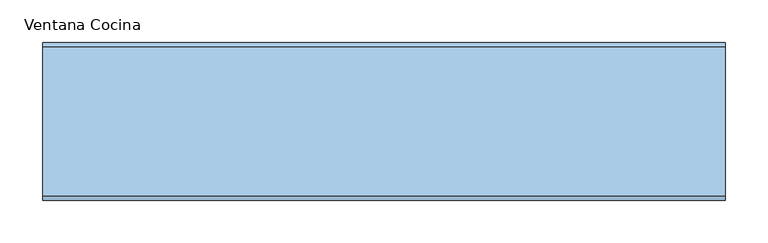
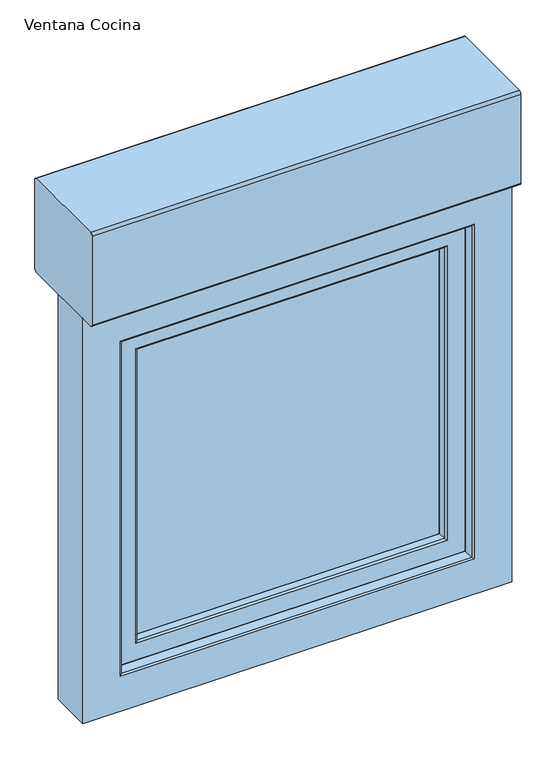
"""IFC4 building model written with IfcOpenShell, lengths in millimetres: window geometry, 2019_ES_Ventana_Replus_re80pvc301_10100_box_1-Hoja_con-Compacto : Ventana Cocina."""

from ifc_helpers import new_model, si_unit, point, frame, frame_2d, origin, place, context, project, spatial, polyline, circle_curve, ellipse_curve, trimmed, segment, composite_curve, outline, extrude, source, transform, mapped, element, save
from ifc_brep_helpers import plane_surface, cylinder_surface, advanced_brep


def ventana_cocina_83fcc546(model_context):
    return source(origin(), model_context, "Body", "SolidModel", [
        extrude(outline(composite_curve([segment(trimmed(circle_curve(frame_2d((-55.0, 1615.0)), 5.0), [point((-55.0, 1610.0))], [point((-60.0, 1615.0))], False, "CARTESIAN"), True, "CONTINUOUS"), segment(polyline([(-60.0, 1615.0), (-60.0, 1790.0)]), True, "CONTINUOUS"), segment(trimmed(circle_curve(frame_2d((-55.0, 1790.0)), 5.0), [point((-60.0, 1790.0))], [point((-55.0, 1795.0))], False, "CARTESIAN"), True, "CONTINUOUS"), segment(polyline([(-55.0, 1795.0), (120.0, 1795.0)]), True, "CONTINUOUS"), segment(trimmed(circle_curve(frame_2d((120.0, 1790.0)), 5.0), [point((120.0, 1795.0))], [point((125.0, 1790.0))], False, "CARTESIAN"), True, "CONTINUOUS"), segment(polyline([(125.0, 1790.0), (125.0, 1615.0)]), True, "CONTINUOUS"), segment(trimmed(circle_curve(frame_2d((120.0, 1615.0)), 5.0), [point((125.0, 1615.0))], [point((120.0, 1610.0))], False, "CARTESIAN"), True, "CONTINUOUS"), segment(polyline([(120.0, 1610.0), (-55.0, 1610.0)]), True, "CONTINUOUS")], self_intersect=False)), frame((-400.0, 0.0, 0.0), z_axis=(1.0, 0.0, 0.0), x_axis=(0.0, 1.0, 0.0)), (0.0, 0.0, 1.0), 800.0),
        extrude(outline(polyline([(78.4999991, 1420.0), (118.4999991, 1420.0), (118.4999991, 1310.0), (98.4999991, 1310.0), (98.4999991, 1400.0), (78.4999991, 1400.0), (78.4999991, 1420.0)])), frame((-334.1999993, 0.0, 0.0), z_axis=(1.0, 0.0, 0.0), x_axis=(0.0, 1.0, 0.0)), (0.0, 0.0, 1.0), 12.0),
        extrude(outline(polyline([(-313.9687607, 78.4999991), (-313.9687607, 68.4999991), (-342.4312378, 68.4999991), (-342.4312378, 78.4999991), (-313.9687607, 78.4999991)])), frame((0.0, 0.0, 1385.217127), z_axis=(0.0, 0.0, 1.0), x_axis=(1.0, 0.0, 0.0)), (0.0, 0.0, 1.0), 49.565746),
        extrude(outline(polyline([(909.8, 297.1999993), (1507.2, 297.1999993), (1507.2, -297.1999993), (909.8, -297.1999993), (909.8, 297.1999993)]), holes=[polyline([(1499.2, 289.1999993), (917.8, 289.1999993), (917.8, -289.1999993), (1499.2, -289.1999993), (1499.2, 289.1999993)])]), frame((0.0, 10.9999999, 0.0), z_axis=(0.0, 1.0, 0.0), x_axis=(0.0, 0.0, 1.0)), (0.0, 0.0, 1.0), 16.0),
        extrude(outline(polyline([(909.8131934, 297.1868058), (1507.1868066, 297.1868058), (1507.1868066, -297.1868058), (909.8131934, -297.1868058), (909.8131934, 297.1868058)]), holes=[polyline([(1499.2, 289.1999993), (917.8, 289.1999993), (917.8, -289.1999993), (1499.2, -289.1999993), (1499.2, 289.1999993)])]), frame((0.0, 31.0000001, 0.0), z_axis=(0.0, 1.0, 0.0), x_axis=(0.0, 0.0, 1.0)), (0.0, 0.0, 1.0), 16.0),
        extrude(outline(polyline([(297.1999993, 6.9999997), (-297.1999993, 6.9999997), (-297.1999993, 10.9999999), (297.1999993, 10.9999999), (297.1999993, 6.9999997)])), frame((0.0, 0.0, 903.7946451), z_axis=(0.0, 0.0, 1.0), x_axis=(1.0, 0.0, 0.0)), (0.0, 0.0, 1.0), 609.4053549),
        extrude(outline(polyline([(297.1999993, 26.9999999), (-297.1999993, 26.9999999), (-297.1999993, 31.0000001), (297.1999993, 31.0000001), (297.1999993, 26.9999999)])), frame((0.0, 0.0, 903.7946451), z_axis=(0.0, 0.0, 1.0), x_axis=(1.0, 0.0, 0.0)), (0.0, 0.0, 1.0), 609.4053549),
        extrude(outline(polyline([(297.1999993, 47.0000001), (-297.1999993, 47.0000001), (-297.1999993, 51.0000003), (297.1999993, 51.0000003), (297.1999993, 47.0000001)])), frame((0.0, 0.0, 903.7946451), z_axis=(0.0, 0.0, 1.0), x_axis=(1.0, 0.0, 0.0)), (0.0, 0.0, 1.0), 609.4053549),
        advanced_brep(
        [(287.2913171, -9.2764571, 1497.2913178), (287.2913171, -9.2764571, 922.7086822), (290.1890946, -11.5, 919.8109047), (290.1890946, -11.5, 1500.1890953), (330.1999993, -11.5, 879.8), (330.1999993, -11.5, 1540.2), (-330.1999993, -11.5, 1540.2), (-330.1999993, -11.5, 879.8), (-290.1890946, -11.5, 919.8109047), (-290.1890946, -11.5, 1500.1890953), (-287.2913171, -9.2764571, 922.7086822), (284.1757968, 2.3508228, 1494.1757976), (284.1757968, 2.3508228, 925.8242024), (-284.1757968, 2.3508228, 925.8242024), (284.6739305, 3.0000033, 1494.6739313), (284.6739305, 3.0000033, 925.3260687), (-284.6739305, 3.0000033, 925.3260687), (291.1999993, 3.0000033, 1501.2), (291.1999993, 3.0000033, 918.8), (-291.1999993, 3.0000033, 918.8), (-291.1999993, 3.0000033, 1501.2), (-284.6739305, 3.0000033, 1494.6739313), (291.1999993, 6.9999997, 1501.2), (291.1999993, 6.9999997, 918.8), (-291.1999993, 6.9999997, 918.8), (311.8162192, 6.9999997, 1521.8162199), (311.8162192, 6.9999997, 898.1837801), (-311.8162192, 6.9999997, 898.1837801), (-311.8162192, 6.9999997, 1521.8162199), (-291.1999993, 6.9999997, 1501.2), (309.1999993, 25.6153717, 1519.2), (309.1999993, 25.6153717, 900.8), (-309.1999993, 25.6153717, 900.8), (309.1999993, 56.4999995, 1519.2), (309.1999993, 56.4999995, 900.8), (-309.1999993, 56.4999995, 900.8), (-309.1999993, 56.4999995, 1519.2), (297.1999993, 56.4999995, 1507.2), (297.1999993, 56.4999995, 912.8), (-297.1999993, 56.4999995, 912.8), (-297.1999993, 56.4999995, 1507.2), (297.1999993, 51.0000003, 1507.2), (297.1999993, 51.0000003, 912.8), (-297.1999993, 51.0000003, 912.8), (-297.1999993, 51.0000003, 1507.2), (286.007687, 51.0000003, 1496.0076877), (286.007687, 51.0000003, 923.9923123), (-286.007687, 51.0000003, 923.9923123), (-286.007687, 51.0000003, 1496.0076877), (285.4940999, 51.6693201, 1495.4941006), (285.4940999, 51.6693201, 924.5058994), (-285.4940999, 51.6693201, 924.5058994), (288.8993918, 64.3780426, 1498.8993925), (288.8993918, 64.3780426, 921.1006075), (-288.8993918, 64.3780426, 921.1006075), (292.6234971, 67.3403297, 1502.6234978), (292.6234971, 67.3403297, 917.3765022), (-292.6234971, 67.3403297, 917.3765022), (305.6488427, 67.7951848, 1515.6488434), (305.6488427, 67.7951848, 904.3511566), (-305.6488427, 67.7951848, 904.3511566), (306.1999993, 67.2629391, 1516.2), (306.1999993, 67.2629391, 903.8), (-306.1999993, 67.2629391, 903.8), (307.4370593, 68.4999991, 1517.43706), (307.4370593, 68.4999991, 902.56294), (-307.4370593, 68.4999991, 902.56294), (360.1999993, 68.4999991, 1570.2), (360.1999993, 68.4999991, 849.8), (-360.1999993, 68.4999991, 849.8), (-360.1999993, 68.4999991, 1570.2), (-307.4370593, 68.4999991, 1517.43706), (363.1999993, 65.4999991, 1573.2), (363.1999993, 65.4999991, 846.8), (-363.1999993, 65.4999991, 846.8), (363.1999993, 50.0, 1573.2), (363.1999993, 50.0, 846.8), (-363.1999993, 50.0, 846.8), (-363.1999993, 50.0, 1573.2), (343.1999993, 50.0, 1553.2), (343.1999993, 50.0, 866.8), (-343.1999993, 50.0, 866.8), (-343.1999993, 50.0, 1553.2), (343.1999993, 11.9999991, 1553.2), (343.1999993, 11.9999991, 866.8), (-343.1999993, 11.9999991, 866.8), (-343.1999993, 11.9999991, 1553.2), (330.1999993, 11.9999991, 1540.2), (330.1999993, 11.9999991, 879.8), (-330.1999993, 11.9999991, 879.8), (-330.1999993, 11.9999991, 1540.2), (-287.2913171, -9.2764571, 1497.2913178), (-284.1757968, 2.3508228, 1494.1757976), (-309.1999993, 25.6153717, 1519.2), (-285.4940999, 51.6693201, 1495.4941006), (-288.8993918, 64.3780426, 1498.8993925), (-292.6234971, 67.3403297, 1502.6234978), (-305.6488427, 67.7951848, 1515.6488434), (-306.1999993, 67.2629391, 1516.2), (-363.1999993, 65.4999991, 1573.2)],
        [
            (0, 1),
            (1, 2, ellipse_curve(frame((290.1890946, -8.5, 919.8109047), z_axis=(0.7071067811865475, 0.0, 0.7071067811865475), x_axis=(-0.7071067811865474, 0.0, 0.7071067811865476)), 4.2426407, 3.0)),
            (2, 3),
            (3, 0, ellipse_curve(frame((290.1890946, -8.5, 1500.1890953), z_axis=(0.7071067811865475, 0.0, -0.7071067811865475), x_axis=(0.7071067811865474, 0.0, 0.7071067811865476)), 4.2426407, 3.0)),
            (4, 5),
            (5, 6),
            (6, 7),
            (7, 4),
            (2, 8),
            (8, 9),
            (9, 3),
            (1, 10),
            (10, 8, ellipse_curve(frame((-290.1890946, -8.5, 919.8109047), z_axis=(0.7071067811865475, 0.0, -0.7071067811865475), x_axis=(0.7071067811865476, 0.0, 0.7071067811865474)), 4.2426407, 3.0)),
            (11, 12),
            (12, 1),
            (0, 11),
            (12, 13),
            (13, 10),
            (14, 15),
            (15, 12, ellipse_curve(frame((284.6739305, 2.4842973, 925.3260687), z_axis=(0.7071067811865475, 0.0, 0.7071067811865475), x_axis=(-0.7071067811865474, 0.0, 0.7071067811865476)), 0.7293184, 0.515706)),
            (11, 14, ellipse_curve(frame((284.6739305, 2.4842973, 1494.6739313), z_axis=(0.7071067811865475, 0.0, -0.7071067811865475), x_axis=(0.7071067811865474, 0.0, 0.7071067811865476)), 0.7293184, 0.515706)),
            (15, 16),
            (16, 13, ellipse_curve(frame((-284.6739305, 2.4842973, 925.3260687), z_axis=(0.7071067811865475, 0.0, -0.7071067811865475), x_axis=(0.7071067811865476, 0.0, 0.7071067811865474)), 0.7293184, 0.515706)),
            (17, 18),
            (18, 19),
            (19, 20),
            (20, 17),
            (14, 21),
            (21, 16),
            (22, 23),
            (23, 18),
            (17, 22),
            (23, 24),
            (24, 19),
            (25, 26),
            (26, 27),
            (27, 28),
            (28, 25),
            (22, 29),
            (29, 24),
            (30, 31),
            (31, 26),
            (25, 30),
            (31, 32),
            (32, 27),
            (33, 34),
            (34, 31),
            (30, 33),
            (34, 35),
            (35, 32),
            (33, 36),
            (36, 35),
            (37, 38),
            (38, 39),
            (39, 40),
            (40, 37),
            (41, 42),
            (42, 38),
            (37, 41),
            (42, 43),
            (43, 39),
            (41, 44),
            (44, 43),
            (45, 46),
            (46, 47),
            (47, 48),
            (48, 45),
            (49, 50),
            (50, 46, ellipse_curve(frame((286.007687, 51.5317048, 923.9923123), z_axis=(0.7071067811865475, 0.0, 0.7071067811865475), x_axis=(-0.7071067811865474, 0.0, 0.7071067811865476)), 0.7519437, 0.5317045)),
            (45, 49, ellipse_curve(frame((286.007687, 51.5317048, 1496.0076877), z_axis=(0.7071067811865475, 0.0, -0.7071067811865475), x_axis=(0.7071067811865474, 0.0, 0.7071067811865476)), 0.7519437, 0.5317045)),
            (50, 51),
            (51, 47, ellipse_curve(frame((-286.007687, 51.5317048, 923.9923123), z_axis=(0.7071067811865475, 0.0, -0.7071067811865475), x_axis=(0.7071067811865476, 0.0, 0.7071067811865474)), 0.7519437, 0.5317045)),
            (52, 53),
            (53, 50),
            (49, 52),
            (53, 54),
            (54, 51),
            (55, 56),
            (56, 53, ellipse_curve(frame((292.7630951, 63.3427664, 917.2369042), z_axis=(0.7071067811865475, 0.0, 0.7071067811865475), x_axis=(-0.7071067811865474, 0.0, 0.7071067811865476)), 5.6568542, 4.0)),
            (52, 55, ellipse_curve(frame((292.7630951, 63.3427664, 1502.7630958), z_axis=(0.7071067811865475, 0.0, -0.7071067811865475), x_axis=(0.7071067811865474, 0.0, 0.7071067811865476)), 5.6568542, 4.0)),
            (56, 57),
            (57, 54, ellipse_curve(frame((-292.7630951, 63.3427664, 917.2369042), z_axis=(0.7071067811865475, 0.0, -0.7071067811865475), x_axis=(0.7071067811865476, 0.0, 0.7071067811865474)), 5.6568542, 4.0)),
            (58, 59),
            (59, 56),
            (55, 58),
            (59, 60),
            (60, 57),
            (61, 62),
            (62, 59, ellipse_curve(frame((305.6674291, 67.2629391, 904.3325701), z_axis=(0.7071067811865475, 0.0, 0.7071067811865475), x_axis=(-0.7071067811865474, 0.0, 0.7071067811865476)), 0.7531679, 0.5325701)),
            (58, 61, ellipse_curve(frame((305.6674291, 67.2629391, 1515.6674299), z_axis=(0.7071067811865475, 0.0, -0.7071067811865475), x_axis=(0.7071067811865474, 0.0, 0.7071067811865476)), 0.7531679, 0.5325701)),
            (62, 63),
            (63, 60, ellipse_curve(frame((-305.6674291, 67.2629391, 904.3325701), z_axis=(0.7071067811865475, 0.0, -0.7071067811865475), x_axis=(0.7071067811865476, 0.0, 0.7071067811865474)), 0.7531679, 0.5325701)),
            (64, 65),
            (65, 62, ellipse_curve(frame((307.4370593, 67.2629391, 902.56294), z_axis=(0.7071067811865475, 0.0, 0.7071067811865475), x_axis=(-0.7071067811865474, 0.0, 0.7071067811865476)), 1.7494671, 1.23706)),
            (61, 64, ellipse_curve(frame((307.4370593, 67.2629391, 1517.43706), z_axis=(0.7071067811865475, 0.0, -0.7071067811865475), x_axis=(0.7071067811865474, 0.0, 0.7071067811865476)), 1.7494671, 1.23706)),
            (65, 66),
            (66, 63, ellipse_curve(frame((-307.4370593, 67.2629391, 902.56294), z_axis=(0.7071067811865475, 0.0, -0.7071067811865475), x_axis=(0.7071067811865476, 0.0, 0.7071067811865474)), 1.7494671, 1.23706)),
            (67, 68),
            (68, 69),
            (69, 70),
            (70, 67),
            (64, 71),
            (71, 66),
            (72, 73),
            (73, 68, ellipse_curve(frame((360.1999993, 65.4999991, 849.8), z_axis=(0.7071067811865475, 0.0, 0.7071067811865475), x_axis=(-0.7071067811865474, 0.0, 0.7071067811865476)), 4.2426407, 3.0)),
            (67, 72, ellipse_curve(frame((360.1999993, 65.4999991, 1570.2), z_axis=(0.7071067811865475, 0.0, -0.7071067811865475), x_axis=(0.7071067811865474, 0.0, 0.7071067811865476)), 4.2426407, 3.0)),
            (73, 74),
            (74, 69, ellipse_curve(frame((-360.1999993, 65.4999991, 849.8), z_axis=(0.7071067811865475, 0.0, -0.7071067811865475), x_axis=(0.7071067811865476, 0.0, 0.7071067811865474)), 4.2426407, 3.0)),
            (75, 76),
            (76, 73),
            (72, 75),
            (76, 77),
            (77, 74),
            (75, 78),
            (78, 77),
            (79, 80),
            (80, 81),
            (81, 82),
            (82, 79),
            (79, 83),
            (83, 84),
            (84, 80),
            (84, 85),
            (85, 81),
            (83, 86),
            (86, 85),
            (87, 88),
            (88, 89),
            (89, 90),
            (90, 87),
            (87, 5),
            (4, 88),
            (7, 89),
            (10, 91),
            (91, 9, ellipse_curve(frame((-290.1890946, -8.5, 1500.1890953), z_axis=(-0.7071067811865475, 0.0, -0.7071067811865475), x_axis=(0.7071067811865474, 0.0, -0.7071067811865476)), 4.2426407, 3.0)),
            (13, 92),
            (92, 91),
            (21, 92, ellipse_curve(frame((-284.6739305, 2.4842973, 1494.6739313), z_axis=(-0.7071067811865475, 0.0, -0.7071067811865475), x_axis=(0.7071067811865474, 0.0, -0.7071067811865476)), 0.7293184, 0.515706)),
            (29, 20),
            (32, 93),
            (93, 28),
            (36, 93),
            (44, 40),
            (51, 94),
            (94, 48, ellipse_curve(frame((-286.007687, 51.5317048, 1496.0076877), z_axis=(-0.7071067811865475, 0.0, -0.7071067811865475), x_axis=(0.7071067811865474, 0.0, -0.7071067811865476)), 0.7519437, 0.5317045)),
            (54, 95),
            (95, 94),
            (57, 96),
            (96, 95, ellipse_curve(frame((-292.7630951, 63.3427664, 1502.7630958), z_axis=(-0.7071067811865475, 0.0, -0.7071067811865475), x_axis=(0.7071067811865474, 0.0, -0.7071067811865476)), 5.6568542, 4.0)),
            (60, 97),
            (97, 96),
            (63, 98),
            (98, 97, ellipse_curve(frame((-305.6674291, 67.2629391, 1515.6674299), z_axis=(-0.7071067811865475, 0.0, -0.7071067811865475), x_axis=(0.7071067811865474, 0.0, -0.7071067811865476)), 0.7531679, 0.5325701)),
            (71, 98, ellipse_curve(frame((-307.4370593, 67.2629391, 1517.43706), z_axis=(-0.7071067811865475, 0.0, -0.7071067811865475), x_axis=(0.7071067811865474, 0.0, -0.7071067811865476)), 1.7494671, 1.23706)),
            (74, 99),
            (99, 70, ellipse_curve(frame((-360.1999993, 65.4999991, 1570.2), z_axis=(-0.7071067811865475, 0.0, -0.7071067811865475), x_axis=(0.7071067811865474, 0.0, -0.7071067811865476)), 4.2426407, 3.0)),
            (78, 99),
            (86, 82),
            (6, 90),
            (91, 0),
            (92, 11),
            (93, 30),
            (94, 49),
            (95, 52),
            (96, 55),
            (97, 58),
            (98, 61),
            (99, 72),
        ],
        [
            cylinder_surface(frame((290.1890946, -8.5, 1573.2), z_axis=(0.0, 0.0, 1.0), x_axis=(-1.0, 0.0, 0.0)), 3.0),
            plane_surface(frame((-330.1999993, -11.5, 1540.2), z_axis=(0.0, -1.0, 0.0), x_axis=(1.0, 0.0, 0.0))),
            cylinder_surface(frame((363.1999993, -8.5, 919.8109047), z_axis=(1.0, 0.0, 0.0), x_axis=(0.0, 0.0, 1.0)), 3.0),
            plane_surface(frame((287.2913171, -9.2764571, 1497.2913178), z_axis=(-0.9659258263570556, -0.258819044848789, 0.0), x_axis=(0.0, 0.0, -1.0))),
            plane_surface(frame((287.2913171, -9.2764571, 922.7086822), z_axis=(0.0, -0.2588190448487859, 0.9659258263570565), x_axis=(-1.0, 0.0, 0.0))),
            cylinder_surface(frame((284.6739305, 2.4842973, 1573.2), z_axis=(0.0, 0.0, 1.0), x_axis=(-1.0, 0.0, 0.0)), 0.515706),
            cylinder_surface(frame((363.1999993, 2.4842973, 925.3260687), z_axis=(1.0, 0.0, 0.0), x_axis=(0.0, 0.0, 1.0)), 0.515706),
            plane_surface(frame((-284.6739305, 3.0000033, 1494.6739313), z_axis=(0.0, 1.0, 0.0), x_axis=(1.0, 0.0, 0.0))),
            plane_surface(frame((291.1999993, 3.0000033, 1501.2), z_axis=(-1.0, 0.0, 0.0), x_axis=(0.0, 0.0, -1.0))),
            plane_surface(frame((291.1999993, 3.0000033, 918.8), z_axis=(0.0, 0.0, 1.0), x_axis=(-1.0, 0.0, 0.0))),
            plane_surface(frame((-291.1999993, 6.9999997, 1501.2), z_axis=(0.0, 1.0, 0.0), x_axis=(1.0, 0.0, 0.0))),
            plane_surface(frame((311.8162192, 6.9999997, 1521.8162199), z_axis=(-0.9902680687415736, -0.13917310096004265, 0.0), x_axis=(0.0, 0.0, -1.0))),
            plane_surface(frame((311.8162192, 6.9999997, 898.1837801), z_axis=(0.0, -0.13917310096003943, 0.990268068741574), x_axis=(-1.0, 0.0, 0.0))),
            plane_surface(frame((309.1999993, 25.6153717, 1519.2), z_axis=(-1.0, 0.0, 0.0), x_axis=(0.0, 0.0, -1.0))),
            plane_surface(frame((309.1999993, 25.6153717, 900.8), z_axis=(0.0, 0.0, 1.0), x_axis=(-1.0, 0.0, 0.0))),
            plane_surface(frame((-309.1999993, 56.4999995, 1519.2), z_axis=(0.0, -1.0, 0.0), x_axis=(1.0, 0.0, 0.0))),
            plane_surface(frame((297.1999993, 56.4999995, 1507.2), z_axis=(1.0, 0.0, 0.0), x_axis=(0.0, 0.0, -1.0))),
            plane_surface(frame((297.1999993, 56.4999995, 912.8), z_axis=(0.0, 0.0, -1.0), x_axis=(-1.0, 0.0, 0.0))),
            plane_surface(frame((-297.1999993, 51.0000003, 1507.2), z_axis=(0.0, -1.0, 0.0), x_axis=(1.0, 0.0, 0.0))),
            cylinder_surface(frame((286.007687, 51.5317048, 1573.2), z_axis=(0.0, 0.0, 1.0), x_axis=(-1.0, 0.0, 0.0)), 0.5317045),
            cylinder_surface(frame((363.1999993, 51.5317048, 923.9923123), z_axis=(1.0, 0.0, 0.0), x_axis=(0.0, 0.0, 1.0)), 0.5317045),
            plane_surface(frame((285.4940999, 51.6693201, 1495.4941006), z_axis=(-0.9659258262890666, 0.2588190451025272, 0.0), x_axis=(0.0, 0.0, -1.0))),
            plane_surface(frame((285.4940999, 51.6693201, 924.5058994), z_axis=(0.0, 0.2588190451025303, 0.9659258262890658), x_axis=(-1.0, 0.0, 0.0))),
            cylinder_surface(frame((292.7630951, 63.3427664, 1573.2), z_axis=(0.0, 0.0, 1.0), x_axis=(-1.0, 0.0, 0.0)), 4.0),
            cylinder_surface(frame((363.1999993, 63.3427664, 917.2369042), z_axis=(1.0, 0.0, 0.0), x_axis=(0.0, 0.0, 1.0)), 4.0),
            plane_surface(frame((292.6234971, 67.3403297, 1502.6234978), z_axis=(-0.03489949670250791, 0.9993908270190955, 0.0), x_axis=(0.0, 0.0, -1.0))),
            plane_surface(frame((292.6234971, 67.3403297, 917.3765022), z_axis=(0.0, 0.9993908270190957, 0.034899496702504675), x_axis=(-1.0, 0.0, 0.0))),
            cylinder_surface(frame((305.6674291, 67.2629391, 1573.2), z_axis=(0.0, 0.0, 1.0), x_axis=(-1.0, 0.0, 0.0)), 0.5325701),
            cylinder_surface(frame((363.1999993, 67.2629391, 904.3325701), z_axis=(1.0, 0.0, 0.0), x_axis=(0.0, 0.0, 1.0)), 0.5325701),
            cylinder_surface(frame((307.4370593, 67.2629391, 1573.2), z_axis=(0.0, 0.0, 1.0), x_axis=(-1.0, 0.0, 0.0)), 1.23706),
            cylinder_surface(frame((363.1999993, 67.2629391, 902.56294), z_axis=(1.0, 0.0, 0.0), x_axis=(0.0, 0.0, 1.0)), 1.23706),
            plane_surface(frame((-307.4370593, 68.4999991, 1517.43706), z_axis=(0.0, 1.0, 0.0), x_axis=(1.0, 0.0, 0.0))),
            cylinder_surface(frame((360.1999993, 65.4999991, 1573.2), z_axis=(0.0, 0.0, 1.0), x_axis=(-1.0, 0.0, 0.0)), 3.0),
            cylinder_surface(frame((363.1999993, 65.4999991, 849.8), z_axis=(1.0, 0.0, 0.0), x_axis=(0.0, 0.0, 1.0)), 3.0),
            plane_surface(frame((363.1999993, 65.4999991, 1573.2), z_axis=(1.0, 0.0, 0.0), x_axis=(0.0, 0.0, -1.0))),
            plane_surface(frame((363.1999993, 65.4999991, 846.8), z_axis=(0.0, 0.0, -1.0), x_axis=(-1.0, 0.0, 0.0))),
            plane_surface(frame((-359.2000019, 50.0, 1569.2000027), z_axis=(0.0, -1.0, 0.0), x_axis=(1.0, 0.0, 0.0))),
            plane_surface(frame((343.1999993, 45.0999991, 1553.2), z_axis=(1.0, 0.0, 0.0), x_axis=(0.0, 0.0, -1.0))),
            plane_surface(frame((343.1999993, 45.0999991, 866.8), z_axis=(0.0, 0.0, -1.0), x_axis=(-1.0, 0.0, 0.0))),
            plane_surface(frame((-335.7000002, 11.9999991, 1545.7000009), z_axis=(0.0, -1.0, 0.0), x_axis=(1.0, 0.0, 0.0))),
            plane_surface(frame((330.1999993, 1.4999991, 1540.2), z_axis=(1.0, 0.0, 0.0), x_axis=(0.0, 0.0, -1.0))),
            plane_surface(frame((330.1999993, 1.4999991, 879.8), z_axis=(0.0, 0.0, -1.0), x_axis=(-1.0, 0.0, 0.0))),
            cylinder_surface(frame((-290.1890946, -8.5, 846.8), z_axis=(0.0, 0.0, -1.0), x_axis=(1.0, 0.0, 0.0)), 3.0),
            plane_surface(frame((-287.2913171, -9.2764571, 922.7086822), z_axis=(0.9659258263570573, -0.25881904484878276, 0.0), x_axis=(0.0, 0.0, 1.0))),
            cylinder_surface(frame((-284.6739305, 2.4842973, 846.8), z_axis=(0.0, 0.0, -1.0), x_axis=(1.0, 0.0, 0.0)), 0.515706),
            plane_surface(frame((-291.1999993, 3.0000033, 918.8), z_axis=(1.0, 0.0, 0.0), x_axis=(0.0, 0.0, 1.0))),
            plane_surface(frame((-311.8162192, 6.9999997, 898.1837801), z_axis=(0.9902680687415745, -0.1391731009600362, 0.0), x_axis=(0.0, 0.0, 1.0))),
            plane_surface(frame((-309.1999993, 25.6153717, 900.8), z_axis=(1.0, 0.0, 0.0), x_axis=(0.0, 0.0, 1.0))),
            plane_surface(frame((-297.1999993, 56.4999995, 912.8), z_axis=(-1.0, 0.0, 0.0), x_axis=(0.0, 0.0, 1.0))),
            cylinder_surface(frame((-286.007687, 51.5317048, 846.8), z_axis=(0.0, 0.0, -1.0), x_axis=(1.0, 0.0, 0.0)), 0.5317045),
            plane_surface(frame((-285.4940999, 51.6693201, 924.5058994), z_axis=(0.9659258262890649, 0.2588190451025334, 0.0), x_axis=(0.0, 0.0, 1.0))),
            cylinder_surface(frame((-292.7630951, 63.3427664, 846.8), z_axis=(0.0, 0.0, -1.0), x_axis=(1.0, 0.0, 0.0)), 4.0),
            plane_surface(frame((-292.6234971, 67.3403297, 917.3765022), z_axis=(0.03489949670250144, 0.9993908270190958, 0.0), x_axis=(0.0, 0.0, 1.0))),
            cylinder_surface(frame((-305.6674291, 67.2629391, 846.8), z_axis=(0.0, 0.0, -1.0), x_axis=(1.0, 0.0, 0.0)), 0.5325701),
            cylinder_surface(frame((-307.4370593, 67.2629391, 846.8), z_axis=(0.0, 0.0, -1.0), x_axis=(1.0, 0.0, 0.0)), 1.23706),
            cylinder_surface(frame((-360.1999993, 65.4999991, 846.8), z_axis=(0.0, 0.0, -1.0), x_axis=(1.0, 0.0, 0.0)), 3.0),
            plane_surface(frame((-363.1999993, 65.4999991, 846.8), z_axis=(-1.0, 0.0, 0.0), x_axis=(0.0, 0.0, 1.0))),
            plane_surface(frame((-343.1999993, 45.0999991, 866.8), z_axis=(-1.0, 0.0, 0.0), x_axis=(0.0, 0.0, 1.0))),
            plane_surface(frame((-330.1999993, 1.4999991, 879.8), z_axis=(-1.0, 0.0, 0.0), x_axis=(0.0, 0.0, 1.0))),
            cylinder_surface(frame((-363.1999993, -8.5, 1500.1890953), z_axis=(-1.0, 0.0, 0.0), x_axis=(0.0, 0.0, -1.0)), 3.0),
            plane_surface(frame((-287.2913171, -9.2764571, 1497.2913178), z_axis=(0.0, -0.2588190448487859, -0.9659258263570564), x_axis=(1.0, 0.0, 0.0))),
            cylinder_surface(frame((-363.1999993, 2.4842973, 1494.6739313), z_axis=(-1.0, 0.0, 0.0), x_axis=(0.0, 0.0, -1.0)), 0.515706),
            plane_surface(frame((-291.1999993, 3.0000033, 1501.2), z_axis=(0.0, 0.0, -1.0), x_axis=(1.0, 0.0, 0.0))),
            plane_surface(frame((-311.8162192, 6.9999997, 1521.8162199), z_axis=(0.0, -0.13917310096003943, -0.990268068741574), x_axis=(1.0, 0.0, 0.0))),
            plane_surface(frame((-309.1999993, 25.6153717, 1519.2), z_axis=(0.0, 0.0, -1.0), x_axis=(1.0, 0.0, 0.0))),
            plane_surface(frame((-297.1999993, 56.4999995, 1507.2), z_axis=(0.0, 0.0, 1.0), x_axis=(1.0, 0.0, 0.0))),
            cylinder_surface(frame((-363.1999993, 51.5317048, 1496.0076877), z_axis=(-1.0, 0.0, 0.0), x_axis=(0.0, 0.0, -1.0)), 0.5317045),
            plane_surface(frame((-285.4940999, 51.6693201, 1495.4941006), z_axis=(0.0, 0.2588190451025303, -0.9659258262890658), x_axis=(1.0, 0.0, 0.0))),
            cylinder_surface(frame((-363.1999993, 63.3427664, 1502.7630958), z_axis=(-1.0, 0.0, 0.0), x_axis=(0.0, 0.0, -1.0)), 4.0),
            plane_surface(frame((-292.6234971, 67.3403297, 1502.6234978), z_axis=(0.0, 0.9993908270190957, -0.034899496702504675), x_axis=(1.0, 0.0, 0.0))),
            cylinder_surface(frame((-363.1999993, 67.2629391, 1515.6674299), z_axis=(-1.0, 0.0, 0.0), x_axis=(0.0, 0.0, -1.0)), 0.5325701),
            cylinder_surface(frame((-363.1999993, 67.2629391, 1517.43706), z_axis=(-1.0, 0.0, 0.0), x_axis=(0.0, 0.0, -1.0)), 1.23706),
            cylinder_surface(frame((-363.1999993, 65.4999991, 1570.2), z_axis=(-1.0, 0.0, 0.0), x_axis=(0.0, 0.0, -1.0)), 3.0),
            plane_surface(frame((-363.1999993, 65.4999991, 1573.2), z_axis=(0.0, 0.0, 1.0), x_axis=(1.0, 0.0, 0.0))),
            plane_surface(frame((-343.1999993, 45.0999991, 1553.2), z_axis=(0.0, 0.0, 1.0), x_axis=(1.0, 0.0, 0.0))),
            plane_surface(frame((-330.1999993, 1.4999991, 1540.2), z_axis=(0.0, 0.0, 1.0), x_axis=(1.0, 0.0, 0.0))),
        ],
        [
            (0, [[1, 2, 3, 4]]),
            (1, [[5, 6, 7, 8], [-3, 9, 10, 11]]),
            (2, [[12, 13, -9, -2]]),
            (3, [[14, 15, -1, 16]]),
            (4, [[17, 18, -12, -15]]),
            (5, [[19, 20, -14, 21]]),
            (6, [[22, 23, -17, -20]]),
            (7, [[24, 25, 26, 27], [-19, 28, 29, -22]]),
            (8, [[30, 31, -24, 32]]),
            (9, [[33, 34, -25, -31]]),
            (10, [[35, 36, 37, 38], [-30, 39, 40, -33]]),
            (11, [[41, 42, -35, 43]]),
            (12, [[44, 45, -36, -42]]),
            (13, [[46, 47, -41, 48]]),
            (14, [[49, 50, -44, -47]]),
            (15, [[-46, 51, 52, -49], [53, 54, 55, 56]]),
            (16, [[57, 58, -53, 59]]),
            (17, [[60, 61, -54, -58]]),
            (18, [[-57, 62, 63, -60], [64, 65, 66, 67]]),
            (19, [[68, 69, -64, 70]]),
            (20, [[71, 72, -65, -69]]),
            (21, [[73, 74, -68, 75]]),
            (22, [[76, 77, -71, -74]]),
            (23, [[78, 79, -73, 80]]),
            (24, [[81, 82, -76, -79]]),
            (25, [[83, 84, -78, 85]]),
            (26, [[86, 87, -81, -84]]),
            (27, [[88, 89, -83, 90]]),
            (28, [[91, 92, -86, -89]]),
            (29, [[93, 94, -88, 95]]),
            (30, [[96, 97, -91, -94]]),
            (31, [[98, 99, 100, 101], [-93, 102, 103, -96]]),
            (32, [[104, 105, -98, 106]]),
            (33, [[107, 108, -99, -105]]),
            (34, [[109, 110, -104, 111]]),
            (35, [[112, 113, -107, -110]]),
            (36, [[-109, 114, 115, -112], [116, 117, 118, 119]]),
            (37, [[120, 121, 122, -116]]),
            (38, [[123, 124, -117, -122]]),
            (39, [[-121, 125, 126, -123], [127, 128, 129, 130]]),
            (40, [[131, -5, 132, -127]]),
            (41, [[-8, 133, -128, -132]]),
            (42, [[134, 135, -10, -13]]),
            (43, [[136, 137, -134, -18]]),
            (44, [[-29, 138, -136, -23]]),
            (45, [[-40, 139, -26, -34]]),
            (46, [[140, 141, -37, -45]]),
            (47, [[-52, 142, -140, -50]]),
            (48, [[-63, 143, -55, -61]]),
            (49, [[144, 145, -66, -72]]),
            (50, [[146, 147, -144, -77]]),
            (51, [[148, 149, -146, -82]]),
            (52, [[150, 151, -148, -87]]),
            (53, [[152, 153, -150, -92]]),
            (54, [[-103, 154, -152, -97]]),
            (55, [[155, 156, -100, -108]]),
            (56, [[-115, 157, -155, -113]]),
            (57, [[-126, 158, -118, -124]]),
            (58, [[-7, 159, -129, -133]]),
            (59, [[160, -4, -11, -135]]),
            (60, [[161, -16, -160, -137]]),
            (61, [[-28, -21, -161, -138]]),
            (62, [[-39, -32, -27, -139]]),
            (63, [[162, -43, -38, -141]]),
            (64, [[-51, -48, -162, -142]]),
            (65, [[-62, -59, -56, -143]]),
            (66, [[163, -70, -67, -145]]),
            (67, [[164, -75, -163, -147]]),
            (68, [[165, -80, -164, -149]]),
            (69, [[166, -85, -165, -151]]),
            (70, [[167, -90, -166, -153]]),
            (71, [[-102, -95, -167, -154]]),
            (72, [[168, -106, -101, -156]]),
            (73, [[-114, -111, -168, -157]]),
            (74, [[-125, -120, -119, -158]]),
            (75, [[-6, -131, -130, -159]]),
        ],
    ),
        advanced_brep(
        [(323.2673545, -12.758819, 1533.2673545), (323.2673545, -12.758819, 886.7326455), (327.2913185, -27.7764571, 882.7086815), (327.2913185, -27.7764571, 1537.2913185), (330.189096, -30.0, 879.810904), (330.189096, -30.0, 1540.189096), (-323.2673545, -12.758819, 886.7326455), (-327.2913185, -27.7764571, 882.7086815), (324.2332803, -11.5, 1534.2332803), (324.2332803, -11.5, 885.7667197), (400.0, -30.0, 1610.0), (400.0, -30.0, 810.0), (400.0, 50.0, 810.0), (400.0, 50.0, 1610.0), (-400.0, 50.0, 810.0), (-400.0, 50.0, 1610.0), (356.1999993, 50.0, 853.8000007), (356.1999993, 50.0, 1566.1999993), (-356.1999993, 50.0, 1566.1999993), (-356.1999993, 50.0, 853.8000007), (-400.0, -30.0, 810.0), (-400.0, -30.0, 1610.0), (-330.189096, -30.0, 879.810904), (-330.189096, -30.0, 1540.189096), (336.1891471, 8.0, 1546.1891471), (336.1891471, 8.0, 873.8108529), (336.1891471, -11.5, 873.8108529), (336.1891471, -11.5, 1546.1891471), (-336.1891471, -11.5, 873.8108529), (-336.1891471, -11.5, 1546.1891471), (-324.2332803, -11.5, 1534.2332803), (-324.2332803, -11.5, 885.7667197), (-336.1891471, 8.0, 873.8108529), (355.1999993, 8.0, 1565.1999993), (355.1999993, 8.0, 854.8000007), (-355.1999993, 8.0, 854.8000007), (-355.1999993, 8.0, 1565.1999993), (-336.1891471, 8.0, 1546.1891471), (355.1999993, 49.0, 854.8000007), (355.1999993, 49.0, 1565.1999993), (-355.1999993, 49.0, 854.8000007), (-323.2673545, -12.758819, 1533.2673545), (-327.2913185, -27.7764571, 1537.2913185), (-355.1999993, 49.0, 1565.1999993)],
        [
            (0, 1),
            (1, 2),
            (2, 3),
            (3, 0),
            (2, 4, ellipse_curve(frame((330.189096, -27.0, 879.810904), z_axis=(0.7071067811865475, 0.0, 0.7071067811865475), x_axis=(-0.7071067811865474, 0.0, 0.7071067811865476)), 4.2426407, 3.0)),
            (4, 5),
            (5, 3, ellipse_curve(frame((330.189096, -27.0, 1540.189096), z_axis=(0.7071067811865475, 0.0, -0.7071067811865475), x_axis=(0.7071067811865474, 0.0, 0.7071067811865476)), 4.2426407, 3.0)),
            (1, 6),
            (6, 7),
            (7, 2),
            (8, 9),
            (9, 1, ellipse_curve(frame((324.2332803, -12.5, 885.7667197), z_axis=(0.7071067811865475, 0.0, 0.7071067811865475), x_axis=(-0.7071067811865474, 0.0, 0.7071067811865476)), 1.4142136, 1.0)),
            (0, 8, ellipse_curve(frame((324.2332803, -12.5, 1534.2332803), z_axis=(0.7071067811865475, 0.0, -0.7071067811865475), x_axis=(0.7071067811865474, 0.0, 0.7071067811865476)), 1.4142136, 1.0)),
            (10, 11),
            (11, 12),
            (12, 13),
            (13, 10),
            (12, 14),
            (14, 15),
            (15, 13),
            (16, 17),
            (17, 18),
            (18, 19),
            (19, 16),
            (11, 20),
            (20, 14),
            (10, 21),
            (21, 20),
            (4, 22),
            (22, 23),
            (23, 5),
            (24, 25),
            (25, 26),
            (26, 27),
            (27, 24),
            (26, 28),
            (28, 29),
            (29, 27),
            (8, 30),
            (30, 31),
            (31, 9),
            (25, 32),
            (32, 28),
            (33, 34),
            (34, 35),
            (35, 36),
            (36, 33),
            (24, 37),
            (37, 32),
            (16, 38, ellipse_curve(frame((356.1999993, 49.0, 853.8000007), z_axis=(0.7071067811865475, 0.0, 0.7071067811865475), x_axis=(-0.7071067811865474, 0.0, 0.7071067811865476)), 1.4142136, 1.0)),
            (38, 39),
            (39, 17, ellipse_curve(frame((356.1999993, 49.0, 1566.1999993), z_axis=(0.7071067811865475, 0.0, -0.7071067811865475), x_axis=(0.7071067811865474, 0.0, 0.7071067811865476)), 1.4142136, 1.0)),
            (38, 34),
            (33, 39),
            (19, 40, ellipse_curve(frame((-356.1999993, 49.0, 853.8000007), z_axis=(0.7071067811865475, 0.0, -0.7071067811865475), x_axis=(0.7071067811865476, 0.0, 0.7071067811865474)), 1.4142136, 1.0)),
            (40, 38),
            (31, 6, ellipse_curve(frame((-324.2332803, -12.5, 885.7667197), z_axis=(0.7071067811865475, 0.0, -0.7071067811865475), x_axis=(0.7071067811865476, 0.0, 0.7071067811865474)), 1.4142136, 1.0)),
            (7, 22, ellipse_curve(frame((-330.189096, -27.0, 879.810904), z_axis=(0.7071067811865475, 0.0, -0.7071067811865475), x_axis=(0.7071067811865476, 0.0, 0.7071067811865474)), 4.2426407, 3.0)),
            (6, 41),
            (41, 42),
            (42, 7),
            (21, 15),
            (37, 29),
            (40, 35),
            (18, 43, ellipse_curve(frame((-356.1999993, 49.0, 1566.1999993), z_axis=(-0.7071067811865475, 0.0, -0.7071067811865475), x_axis=(0.7071067811865474, 0.0, -0.7071067811865476)), 1.4142136, 1.0)),
            (43, 40),
            (30, 41, ellipse_curve(frame((-324.2332803, -12.5, 1534.2332803), z_axis=(-0.7071067811865475, 0.0, -0.7071067811865475), x_axis=(0.7071067811865474, 0.0, -0.7071067811865476)), 1.4142136, 1.0)),
            (42, 23, ellipse_curve(frame((-330.189096, -27.0, 1540.189096), z_axis=(-0.7071067811865475, 0.0, -0.7071067811865475), x_axis=(0.7071067811865474, 0.0, -0.7071067811865476)), 4.2426407, 3.0)),
            (43, 36),
            (41, 0),
            (3, 42),
            (39, 43),
        ],
        [
            plane_surface(frame((327.2913185, -27.7764571, 1537.2913185), z_axis=(-0.9659258262890693, -0.25881904510251696, 0.0), x_axis=(0.0, 0.0, -1.0))),
            cylinder_surface(frame((330.189096, -27.0, 1610.0), z_axis=(0.0, 0.0, 1.0), x_axis=(-1.0, 0.0, 0.0)), 3.0),
            plane_surface(frame((327.2913185, -27.7764571, 882.7086815), z_axis=(0.0, -0.25881904510251386, 0.9659258262890702), x_axis=(-1.0, 0.0, 0.0))),
            cylinder_surface(frame((324.2332803, -12.5, 1610.0), z_axis=(0.0, 0.0, 1.0), x_axis=(-1.0, 0.0, 0.0)), 1.0),
            plane_surface(frame((400.0, 50.0, 1610.0), z_axis=(1.0, 0.0, 0.0), x_axis=(0.0, 0.0, -1.0))),
            plane_surface(frame((-356.1999993, 50.0, 1566.1999993), z_axis=(0.0, 1.0, 0.0), x_axis=(1.0, 0.0, 0.0))),
            plane_surface(frame((400.0, 50.0, 810.0), z_axis=(0.0, 0.0, -1.0), x_axis=(-1.0, 0.0, 0.0))),
            plane_surface(frame((-400.0, -30.0, 1610.0), z_axis=(0.0, -1.0, 0.0), x_axis=(1.0, 0.0, 0.0))),
            plane_surface(frame((336.1891471, -11.5, 1546.1891471), z_axis=(-1.0, 0.0, 0.0), x_axis=(0.0, 0.0, -1.0))),
            plane_surface(frame((-324.2332803, -11.5, 1534.2332803), z_axis=(0.0, 1.0, 0.0), x_axis=(1.0, 0.0, 0.0))),
            plane_surface(frame((336.1891471, -11.5, 873.8108529), z_axis=(0.0, 0.0, 1.0), x_axis=(-1.0, 0.0, 0.0))),
            plane_surface(frame((-336.1891471, 8.0, 1546.1891471), z_axis=(0.0, 1.0, 0.0), x_axis=(1.0, 0.0, 0.0))),
            cylinder_surface(frame((356.1999993, 49.0, 1610.0), z_axis=(0.0, 0.0, 1.0), x_axis=(-1.0, 0.0, 0.0)), 1.0),
            plane_surface(frame((355.1999993, 8.0, 1565.1999993), z_axis=(-1.0, 0.0, 0.0), x_axis=(0.0, 0.0, -1.0))),
            cylinder_surface(frame((400.0, 49.0, 853.8000007), z_axis=(1.0, 0.0, 0.0), x_axis=(0.0, 0.0, 1.0)), 1.0),
            cylinder_surface(frame((400.0, -12.5, 885.7667197), z_axis=(1.0, 0.0, 0.0), x_axis=(0.0, 0.0, 1.0)), 1.0),
            cylinder_surface(frame((400.0, -27.0, 879.810904), z_axis=(1.0, 0.0, 0.0), x_axis=(0.0, 0.0, 1.0)), 3.0),
            plane_surface(frame((-327.2913185, -27.7764571, 882.7086815), z_axis=(0.9659258262890711, -0.25881904510251075, 0.0), x_axis=(0.0, 0.0, 1.0))),
            plane_surface(frame((-400.0, 50.0, 810.0), z_axis=(-1.0, 0.0, 0.0), x_axis=(0.0, 0.0, 1.0))),
            plane_surface(frame((-336.1891471, -11.5, 873.8108529), z_axis=(1.0, 0.0, 0.0), x_axis=(0.0, 0.0, 1.0))),
            plane_surface(frame((355.1999993, 8.0, 854.8000007), z_axis=(0.0, 0.0, 1.0), x_axis=(-1.0, 0.0, 0.0))),
            cylinder_surface(frame((-356.1999993, 49.0, 810.0), z_axis=(0.0, 0.0, -1.0), x_axis=(1.0, 0.0, 0.0)), 1.0),
            cylinder_surface(frame((-324.2332803, -12.5, 810.0), z_axis=(0.0, 0.0, -1.0), x_axis=(1.0, 0.0, 0.0)), 1.0),
            cylinder_surface(frame((-330.189096, -27.0, 810.0), z_axis=(0.0, 0.0, -1.0), x_axis=(1.0, 0.0, 0.0)), 3.0),
            plane_surface(frame((-355.1999993, 8.0, 854.8000007), z_axis=(1.0, 0.0, 0.0), x_axis=(0.0, 0.0, 1.0))),
            plane_surface(frame((-327.2913185, -27.7764571, 1537.2913185), z_axis=(0.0, -0.25881904510251386, -0.9659258262890702), x_axis=(1.0, 0.0, 0.0))),
            plane_surface(frame((-400.0, 50.0, 1610.0), z_axis=(0.0, 0.0, 1.0), x_axis=(1.0, 0.0, 0.0))),
            plane_surface(frame((-336.1891471, -11.5, 1546.1891471), z_axis=(0.0, 0.0, -1.0), x_axis=(1.0, 0.0, 0.0))),
            cylinder_surface(frame((-400.0, 49.0, 1566.1999993), z_axis=(-1.0, 0.0, 0.0), x_axis=(0.0, 0.0, -1.0)), 1.0),
            cylinder_surface(frame((-400.0, -12.5, 1534.2332803), z_axis=(-1.0, 0.0, 0.0), x_axis=(0.0, 0.0, -1.0)), 1.0),
            cylinder_surface(frame((-400.0, -27.0, 1540.189096), z_axis=(-1.0, 0.0, 0.0), x_axis=(0.0, 0.0, -1.0)), 3.0),
            plane_surface(frame((-355.1999993, 8.0, 1565.1999993), z_axis=(0.0, 0.0, -1.0), x_axis=(1.0, 0.0, 0.0))),
        ],
        [
            (0, [[1, 2, 3, 4]]),
            (1, [[-3, 5, 6, 7]]),
            (2, [[8, 9, 10, -2]]),
            (3, [[11, 12, -1, 13]]),
            (4, [[14, 15, 16, 17]]),
            (5, [[-16, 18, 19, 20], [21, 22, 23, 24]]),
            (6, [[25, 26, -18, -15]]),
            (7, [[-14, 27, 28, -25], [-6, 29, 30, 31]]),
            (8, [[32, 33, 34, 35]]),
            (9, [[-34, 36, 37, 38], [-11, 39, 40, 41]]),
            (10, [[42, 43, -36, -33]]),
            (11, [[44, 45, 46, 47], [-32, 48, 49, -42]]),
            (12, [[-21, 50, 51, 52]]),
            (13, [[-51, 53, -44, 54]]),
            (14, [[-24, 55, 56, -50]]),
            (15, [[-41, 57, -8, -12]]),
            (16, [[-10, 58, -29, -5]]),
            (17, [[59, 60, 61, -9]]),
            (18, [[-28, 62, -19, -26]]),
            (19, [[-49, 63, -37, -43]]),
            (20, [[-56, 64, -45, -53]]),
            (21, [[-23, 65, 66, -55]]),
            (22, [[-40, 67, -59, -57]]),
            (23, [[-61, 68, -30, -58]]),
            (24, [[-66, 69, -46, -64]]),
            (25, [[70, -4, 71, -60]]),
            (26, [[-27, -17, -20, -62]]),
            (27, [[-48, -35, -38, -63]]),
            (28, [[-22, -52, 72, -65]]),
            (29, [[-39, -13, -70, -67]]),
            (30, [[-71, -7, -31, -68]]),
            (31, [[-72, -54, -47, -69]]),
        ],
    ),
    ])


if __name__ == "__main__":
    model = new_model("IFC4")
    model_context = context("Model", 3, world=origin())
    ifc_project = project(units=[si_unit("LENGTHUNIT", "METRE", prefix="MILLI")], contexts=[model_context])
    site = spatial("IfcSite", under=ifc_project)
    building = spatial("IfcBuilding", under=site)
    placement = place(None, origin())
    ventana_cocina_shape = ventana_cocina_83fcc546(model_context)
    element("IfcWindow", 1, ObjectType="2019_ES_Ventana_Replus_re80pvc301_10100_box_1-Hoja_con-Compacto : Ventana Cocina", at=placement, inside=building, context=model_context, shape_type="MappedRepresentation", body=[
        mapped(ventana_cocina_shape, transform((0.0, 0.0, 0.0), x_axis=(1.0, 0.0, 0.0), y_axis=(0.0, 1.0, 0.0), z_axis=(0.0, 0.0, 1.0))),
    ])
    save(model, "model.ifc")

# Revit data of these elements
# Type "2019_ES_Ventana_Replus_re80pvc301_10100_box_1-Hoja_con-Compacto : Ventana Cocina"
#   Type Mark = "41"
#   URL = "https://replus.es/"
#   Product data url = "https://bimetica.com/es/objetos-bim-replus-ventana-practicable-oscilobatiente-una-hoja-con-compacto-9540"
#   Product Guid = ""
#   Model = "10100 BOX"
#   Material secondary = "Glass"
#   Material main = "PVC"
#   Manufacturer = "Replus"
#   Keynote = "08500"
#   EAN code = ""
#   Description = "Perfiles de PVC con triple junta (por junta rígida en el marco). Protegiendo de este modo todos los puntos de cierre y proporcionando una junta perimetral completa, con un grosor en el perfil de 3 mm. Vidrio de alta calidad con diferentes posibilidades"
#   Assembly Code = "B2020100"
#   Analytic Construction = "<None>"
#   Ι_Wll Thcknss [instance default] = 20.0 cm
#   Ι_Wdth Cntrl = 80.0 cm
#   Ι_Nst Cntrl [instance default] = 0.0 cm
#   Ι_Hndl Hght Cntrl = 60.0 cm
#   Ι_Hght Cntrl = 80.0 cm
#   Rough Width = 82.0 cm
#   Rough Height = 82.0 cm
#   Retranqueo [instance default] = 0.0 cm
#   I_Lf_Cntrl = 72.64 cm
#   Hueco = 1.0 cm
#   Height = 80.0 cm
#   Default Sill Height = 80.0 cm
#   Width = 80.0 cm
#   Altura de Manilla = 65.0 cm
#   Visibilidad Líneas Apertura - Planta = yes
#   Visibilidad Líneas Apertura - Alzado = yes
#   Exceso Dimensiones = no
#   Edition number = 1
#   Advertencia Dimensión = yes
#   Product Material = PVC - Replus - 9152 - White
#   Wall Closure = (empty or 0)
# Element 1 (IfcWindow, "2019_ES_Ventana_Replus_re80pvc301_10100_box_1-Hoja_con-Compacto : Ventana Cocina")
#   Ι_Wll Thcknss = 10.0 cm
#   Materials on its faces: "PVC - Replus - 9152 - White", "Rubber - Replus - Black", "Glass - Replus"
# Materials
#   "PVC - Replus - 9152 - White": class "Miscellaneous", colour RGB 174 174 166, transparency 0, Manufacturer = "Replus", Comments = "Rendering appearance not upgraded ", URL = "https://replus.es/", Cost = 0
#   "Rubber - Replus - Black": class "Plastic", colour RGB 63 63 63, transparency 0, Description = "Natural rubber, black", Cost = 0
#   "Glass - Replus": class "Glass", colour RGB 218 227 224, transparency 0.85, Cost = 0
